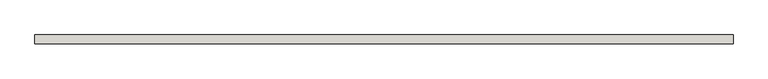
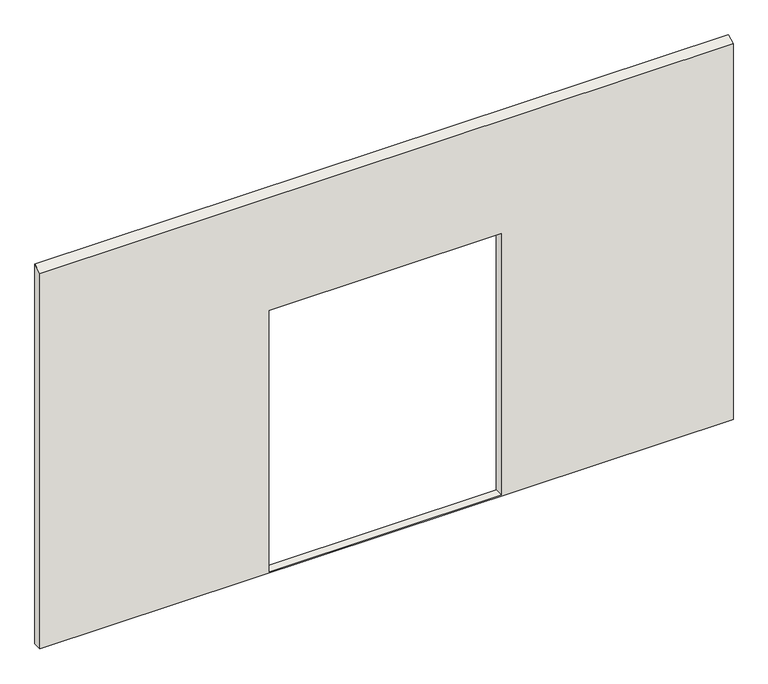
"""IFC4 building model written with IfcOpenShell, lengths in millimetres: wall geometry, 0_3d."""

import ifcopenshell
import ifcopenshell.guid

model = None  # the IFC model being written
_history = None  # IfcOwnerHistory: only IFC2X3 demands one
_inside = {}  # id of a spatial element -> (the spatial element, [elements in it])
_under = {}  # id of a project, library or spatial element -> (it, [spatial elements below it])
_declared = {}  # id of a project -> (the project, [libraries it declares])
_typed = {}  # id of a type object -> (the type object, [elements of that type])
_made_of = {}  # id of a material, layer set ... -> (it, [elements and type objects made of it])


def new_model(schema):
    """Start an empty IFC model of exactly this schema.

    Asked for "IFC4X3", IfcOpenShell would pick the latest addendum, in which some entities
    have other attributes; the version numbers below select the first issue.
    IFC2X3 requires an IfcOwnerHistory on every rooted entity: one is made here for all.
    """
    global model, _history
    if schema == "IFC4X3":
        model = ifcopenshell.file(schema_version=(4, 3, 0, 0))
    else:
        model = ifcopenshell.file(schema=schema)
    _inside.clear()
    _under.clear()
    _declared.clear()
    _typed.clear()
    _made_of.clear()
    _history = None
    if model.schema == "IFC2X3":
        org = make("IfcOrganization", Name="unknown")
        user = make(
            "IfcPersonAndOrganization",
            ThePerson=make("IfcPerson", FamilyName="unknown"),
            TheOrganization=org,
        )
        app = make(
            "IfcApplication",
            ApplicationDeveloper=org,
            Version="unknown",
            ApplicationFullName="unknown",
            ApplicationIdentifier="unknown",
        )
        _history = make(
            "IfcOwnerHistory",
            OwningUser=user,
            OwningApplication=app,
            ChangeAction="ADDED",
            CreationDate=0,
        )
    return model


def make(cls, **values):
    """One entity of the class cls with the attributes given. An attribute that is None is left unset."""
    return model.create_entity(
        cls, **{name: value for name, value in values.items() if value is not None}
    )


def rooted(cls, **values):
    """An entity with a GlobalId (a new one), such as an element, a storey or a relation."""
    return make(cls, GlobalId=ifcopenshell.guid.new(), OwnerHistory=_history, **values)


def si_unit(unit_type, name, prefix=None):
    """IfcSIUnit, for example si_unit("LENGTHUNIT", "METRE", prefix="MILLI")."""
    return make("IfcSIUnit", UnitType=unit_type, Prefix=prefix, Name=name)


def assignment(units):
    """IfcUnitAssignment: the units of a project."""
    return None if units is None else make("IfcUnitAssignment", Units=units)


def point(xyz):
    """IfcCartesianPoint."""
    return None if xyz is None else make("IfcCartesianPoint", Coordinates=xyz)


def direction(xyz):
    """IfcDirection."""
    return None if xyz is None else make("IfcDirection", DirectionRatios=xyz)


def frame(location, z_axis=None, x_axis=None):
    """IfcAxis2Placement3D, a coordinate frame: its origin and axes. An axis left out is left unset."""
    return make(
        "IfcAxis2Placement3D",
        Location=point(location),
        Axis=direction(z_axis),
        RefDirection=direction(x_axis),
    )


def origin():
    """The frame at (0, 0, 0) with its axes left unset."""
    return frame((0.0, 0.0, 0.0))


def place(relative_to, where):
    """IfcLocalPlacement: puts the frame where relative to a parent placement (None: the world)."""
    return make(
        "IfcLocalPlacement", PlacementRelTo=relative_to, RelativePlacement=where
    )


def context(
    kind, dimensions, precision=None, world=None, true_north=None, identifier=None
):
    """IfcGeometricRepresentationContext, for example the 3D "Model" context."""
    return make(
        "IfcGeometricRepresentationContext",
        ContextIdentifier=identifier,
        ContextType=kind,
        CoordinateSpaceDimension=dimensions,
        Precision=precision,
        WorldCoordinateSystem=world,
        TrueNorth=true_north,
    )


def project(units=None, contexts=None):
    """IfcProject with its units and contexts."""
    return rooted(
        "IfcProject",
        Name="project",
        RepresentationContexts=contexts,
        UnitsInContext=assignment(units),
    )


def spatial(cls, under=None, at=None, **own):
    """A site, building, storey or space (cls), placed at a placement, below another one or the project."""
    s = rooted(cls, ObjectPlacement=at, **own)
    if under is not None:
        _under.setdefault(under.id(), (under, []))[1].append(s)
    return s


def faces_of(points, faces, orient=None, outer=None):
    """IfcFace entities. A face is a list of loops; a loop is a list of indices into points, from 0.

    orient and outer hold one flag for each loop. By default every Orientation is true, the
    first loop of a face is its IfcFaceOuterBound and the others are IfcFaceBound.
    """
    made = []
    for i, loops in enumerate(faces):
        bounds = []
        for j, loop in enumerate(loops):
            is_outer = j == 0 if outer is None else outer[i][j]
            bounds.append(
                make(
                    "IfcFaceOuterBound" if is_outer else "IfcFaceBound",
                    Bound=make("IfcPolyLoop", Polygon=[points[k] for k in loop]),
                    Orientation=True if orient is None else orient[i][j],
                )
            )
        made.append(make("IfcFace", Bounds=bounds))
    return made


def faceted_brep(points, faces, orient=None, outer=None, voids=None):
    """IfcFacetedBrep: a solid bounded by flat faces; with voids (closed shells), ...WithVoids."""
    shared = [point(p) for p in points]
    hull = make("IfcClosedShell", CfsFaces=faces_of(shared, faces, orient, outer))
    if voids is None:
        return make("IfcFacetedBrep", Outer=hull)
    return make(
        "IfcFacetedBrepWithVoids",
        Outer=hull,
        Voids=[
            make(cls, CfsFaces=faces_of(shared, fs, o, b)) for cls, fs, o, b in voids
        ],
    )


def shape(context_of_items, identifier, shape_type, items):
    """IfcShapeRepresentation: the items that make up one representation, for example the "Body"."""
    return make(
        "IfcShapeRepresentation",
        ContextOfItems=context_of_items,
        RepresentationIdentifier=identifier,
        RepresentationType=shape_type,
        Items=items,
    )


def source(mapping_origin, context_of_items, identifier, shape_type, items):
    """IfcRepresentationMap: a shape defined once, which mapped items show again and again."""
    return make(
        "IfcRepresentationMap",
        MappingOrigin=mapping_origin,
        MappedRepresentation=shape(context_of_items, identifier, shape_type, items),
    )


def transform(
    local_origin,
    x_axis=None,
    y_axis=None,
    z_axis=None,
    scale=None,
    scale2=None,
    scale3=None,
    uniform=True,
):
    """IfcCartesianTransformationOperator3D, or its non-uniform kind. x_axis, y_axis, z_axis: its Axis1, 2, 3."""
    if uniform:
        return make(
            "IfcCartesianTransformationOperator3D",
            Axis1=direction(x_axis),
            Axis2=direction(y_axis),
            LocalOrigin=point(local_origin),
            Scale=scale,
            Axis3=direction(z_axis),
        )
    return make(
        "IfcCartesianTransformationOperator3DnonUniform",
        Axis1=direction(x_axis),
        Axis2=direction(y_axis),
        LocalOrigin=point(local_origin),
        Scale=scale,
        Axis3=direction(z_axis),
        Scale2=scale2,
        Scale3=scale3,
    )


def mapped(mapping_source, mapping_target):
    """IfcMappedItem: shows the shape of a source again, moved by a transform."""
    return make(
        "IfcMappedItem", MappingSource=mapping_source, MappingTarget=mapping_target
    )


def made_of(thing, what):
    """Note that an element or type object is made of a material, layer set ...; save() writes the relation."""
    if what is not None:
        _made_of.setdefault(what.id(), (what, []))[1].append(thing)
    return thing


def element(
    cls,
    number,
    at=None,
    inside=None,
    cuts=None,
    type_object=None,
    material=None,
    context=None,
    identifier="Body",
    shape_type=None,
    held_by="IfcProductDefinitionShape",
    body=None,
    shapes=None,
    **own,
):
    """One element of the class cls, such as IfcWall. Its Tag is "e" and its number.

    at: its placement. inside: the storey or other place that contains it. cuts: it is an
    opening in that element (IfcRelVoidsElement). A single representation is given by context,
    identifier, shape_type and body (its items); several are given by shapes. held_by: the class
    of the entity that holds the representations. save() writes the other relations.
    """
    e = rooted(cls, Tag="e%d" % number, ObjectPlacement=at, **own)
    if body is not None:
        shapes = [shape(context, identifier, shape_type, body)]
    if shapes is not None:
        e.Representation = make(held_by, Representations=shapes)
    if inside is not None:
        _inside.setdefault(inside.id(), (inside, []))[1].append(e)
    if cuts is not None:
        rooted(
            "IfcRelVoidsElement", RelatingBuildingElement=cuts, RelatedOpeningElement=e
        )
    if type_object is not None:
        _typed.setdefault(type_object.id(), (type_object, []))[1].append(e)
    return made_of(e, material)


def aggregate(whole, parts):
    """IfcRelAggregates: a whole, such as a stair, and the parts it consists of."""
    return rooted("IfcRelAggregates", RelatingObject=whole, RelatedObjects=parts)


def save(model, path):
    """Write the relations noted so far, then the file.

    IfcRelAggregates (storeys below a building ...), IfcRelContainedInSpatialStructure (elements
    in a storey), IfcRelDefinesByType, IfcRelAssociatesMaterial and IfcRelDeclares: one each for
    every whole, place, type object, material and project.
    """
    for whole, parts in _under.values():
        aggregate(whole, parts)
    for where, things in _inside.values():
        rooted(
            "IfcRelContainedInSpatialStructure",
            RelatedElements=things,
            RelatingStructure=where,
        )
    for kind, things in _typed.values():
        rooted("IfcRelDefinesByType", RelatedObjects=things, RelatingType=kind)
    for what, things in _made_of.values():
        rooted("IfcRelAssociatesMaterial", RelatedObjects=things, RelatingMaterial=what)
    for by, libraries in _declared.values():
        rooted("IfcRelDeclares", RelatingContext=by, RelatedDefinitions=libraries)
    model.write(path)


def wall_d0848de2(model_context):
    return source(origin(), model_context, "Body", "Brep", [
        faceted_brep([(1875.0, 70.0, 10.0), (1875.0, 70.0, 2270.0), (1875.0, 0.0, 2270.0), (1875.0, 0.0, 10.0), (3775.0, 70.0, 2270.0), (3775.0, 0.0, 2270.0), (3775.0, 70.0, 10.0), (3775.0, 0.0, 10.0), (5670.0, 0.0, 3247.913011), (5670.0, 70.0, 3283.5797924), (0.0, 70.0, 3283.5797924), (0.0, 0.0, 3247.913011), (0.0, 70.0, 0.0), (0.0, 0.0, 0.0), (5670.0, 0.0, 0.0), (5670.0, 70.0, 0.0)], [[[0, 1, 2, 3]], [[1, 4, 5, 2]], [[4, 6, 7, 5]], [[6, 0, 3, 7]], [[8, 9, 10, 11]], [[11, 10, 12, 13]], [[9, 8, 14, 15]], [[8, 11, 13, 14], [3, 2, 5, 7]], [[15, 12, 10, 9], [1, 0, 6, 4]], [[12, 15, 14, 13]]]),
    ])


if __name__ == "__main__":
    model = new_model("IFC4")
    model_context = context("Model", 3, world=origin())
    ifc_project = project(units=[si_unit("LENGTHUNIT", "METRE", prefix="MILLI")], contexts=[model_context])
    site = spatial("IfcSite", under=ifc_project)
    building = spatial("IfcBuilding", under=site)
    placement = place(None, origin())
    wall_shape = wall_d0848de2(model_context)
    element("IfcWall", 1, ObjectType="0_3d", at=placement, inside=building, context=model_context, shape_type="MappedRepresentation", body=[
        mapped(wall_shape, transform((0.0, 0.0, 0.0), x_axis=(1.0, 0.0, 0.0), y_axis=(0.0, 1.0, 0.0), z_axis=(0.0, 0.0, 1.0))),
    ])
    save(model, "model.ifc")

# Revit data of these elements
# Element 1 (IfcWall, "0_3d")
#   Materials on its faces: "Glass_Simple"
# Materials
#   "Glass_Simple": class "Unassigned", colour RGB 255 255 255, transparency 0.9
